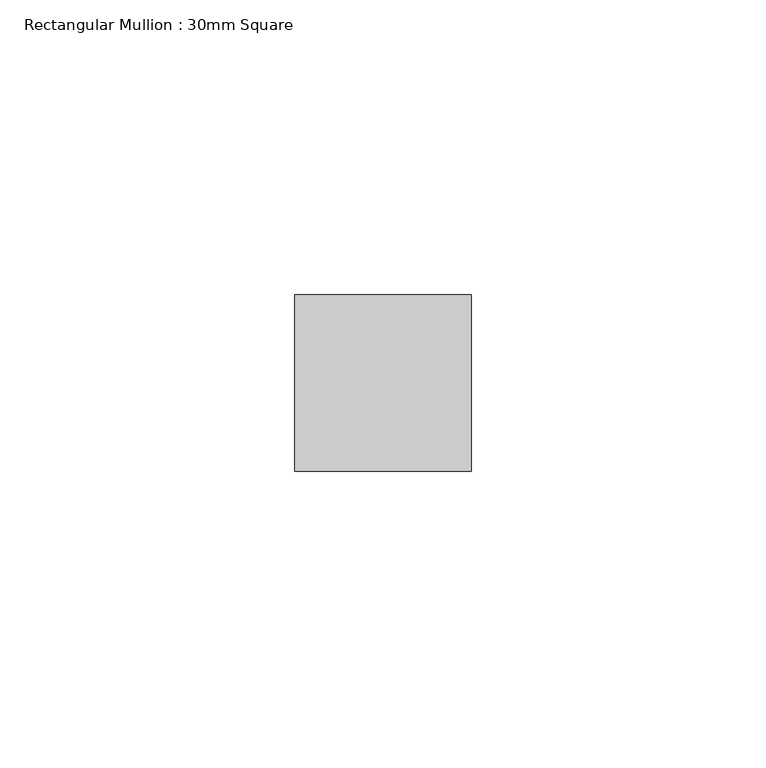
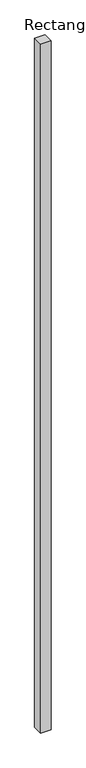
"""IFC4 building model written with IfcOpenShell, lengths in millimetres: member geometry, Rectangular Mullion : 30mm Square."""

from ifc_helpers import new_model, si_unit, frame, origin, place, context, project, spatial, polyline, outline, extrude, source, transform, mapped, element, save


def rectangular_mullion_30mm_square_8c9cc502(model_context):
    return source(origin(), model_context, "Body", "SweptSolid", [
        extrude(outline(polyline([(15.0, 15.0), (15.0, -15.0), (-15.0, -15.0), (-15.0, 15.0), (15.0, 15.0)])), frame((0.0, 0.0, -2093.9136695), z_axis=(0.0, 0.0, 1.0), x_axis=(1.0, 0.0, 0.0)), (0.0, 0.0, 1.0), 2093.9136695),
    ])


if __name__ == "__main__":
    model = new_model("IFC4")
    model_context = context("Model", 3, world=origin())
    ifc_project = project(units=[si_unit("LENGTHUNIT", "METRE", prefix="MILLI")], contexts=[model_context])
    site = spatial("IfcSite", under=ifc_project)
    building = spatial("IfcBuilding", under=site)
    placement = place(None, origin())
    rectangular_mullion_30mm_square_shape = rectangular_mullion_30mm_square_8c9cc502(model_context)
    element("IfcMember", 1, ObjectType="Rectangular Mullion : 30mm Square", at=placement, inside=building, context=model_context, shape_type="MappedRepresentation", body=[
        mapped(rectangular_mullion_30mm_square_shape, transform((0.0, 0.0, 0.0), x_axis=(1.0, 0.0, 0.0), y_axis=(0.0, 1.0, 0.0), z_axis=(0.0, 0.0, 1.0))),
    ])
    save(model, "model.ifc")

# Revit data of these elements
# Type "Rectangular Mullion : 30mm Square"
#   built-in parameter 1007304 = 0.0984252 (stored number, unit not read)
#   built-in parameter 1007301 = 0.0492126 (stored number, unit not read)
#   built-in parameter 1007300 = 0.0492126 (stored number, unit not read)
# Element 1 (IfcMember, "Rectangular Mullion : 30mm Square")
#   Materials on its faces: "Aluminum"
# Materials
#   "Aluminum": class "Metal", colour RGB 244 244 244, transparency 0, Description = "Aluminum 6061", Cost = 0
